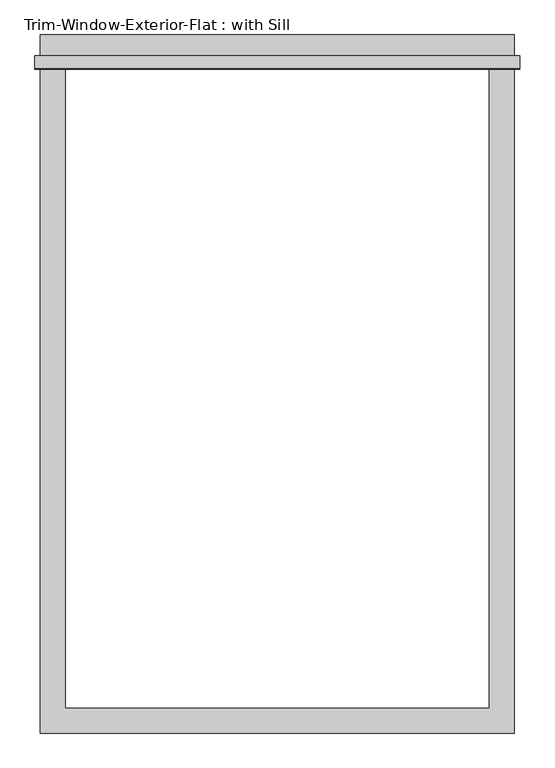
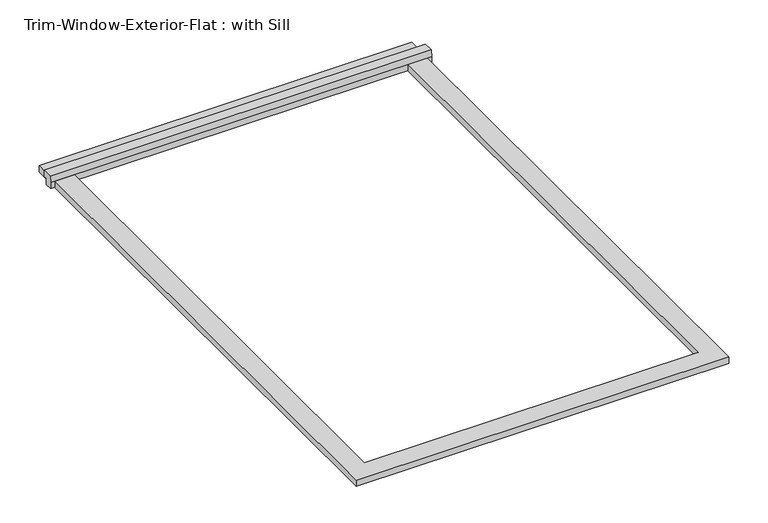
"""IFC4 building model written with IfcOpenShell, lengths in millimetres: proxy geometry, Trim-Window-Exterior-Flat : with Sill."""

from ifc_helpers import new_model, si_unit, frame, origin, origin_with_axes, place, context, project, spatial, polyline, outline, extrude, source, transform, mapped, element, save


def trim_window_exterior_flat_with_sill_c46fdb85(model_context):
    return source(origin(), model_context, "Body", "SweptSolid", [
        extrude(outline(polyline([(546.1, 1495.3823709), (-546.1, 1495.3823709), (-546.1, 1552.5323709), (546.1, 1552.5323709), (546.1, 1495.3823709)])), origin_with_axes(), (0.0, 0.0, 1.0), 19.05),
        extrude(outline(polyline([(1504.95, 38.1), (1504.95, 19.05), (1495.3823709, 19.05), (1495.3823709, 0.0), (1473.2, 0.0), (1473.2, 19.05), (1475.6580645, 38.1), (1504.95, 38.1)])), frame((-558.8, 0.0, 0.0), z_axis=(1.0, 0.0, 0.0), x_axis=(0.0, 1.0, 0.0)), (0.0, 0.0, 1.0), 1117.6),
        extrude(outline(polyline([(-546.1, -57.15), (-546.1, 1473.2), (-488.95, 1473.2), (-488.95, 0.0), (488.95, 0.0), (488.95, 1473.2), (546.1, 1473.2), (546.1, -57.15), (-546.1, -57.15)])), origin_with_axes(), (0.0, 0.0, 1.0), 19.05),
    ])


if __name__ == "__main__":
    model = new_model("IFC4")
    model_context = context("Model", 3, world=origin())
    ifc_project = project(units=[si_unit("LENGTHUNIT", "METRE", prefix="MILLI")], contexts=[model_context])
    site = spatial("IfcSite", under=ifc_project)
    building = spatial("IfcBuilding", under=site)
    placement = place(None, origin())
    trim_window_exterior_flat_with_sill_shape = trim_window_exterior_flat_with_sill_c46fdb85(model_context)
    element("IfcBuildingElementProxy", 1, Name="Trim-Window-Exterior-Flat : with Sill", ObjectType="Trim-Window-Exterior-Flat : with Sill", at=placement, inside=building, context=model_context, shape_type="MappedRepresentation", body=[
        mapped(trim_window_exterior_flat_with_sill_shape, transform((0.0, 0.0, 0.0), x_axis=(1.0, 0.0, 0.0), y_axis=(0.0, 1.0, 0.0), z_axis=(0.0, 0.0, 1.0))),
    ])
    save(model, "model.ifc")

# Revit data of these elements
# Type "Trim-Window-Exterior-Flat : with Sill"
#   Trim Width = 0' - 2 1/4"
#   Trim Thickness_Picture Frame = 0' - 1 1/4"
#   Trim Thickness_with Sill = 0' - 0 3/4"
#   Sill Thickness = 0' - 1 1/4"
#   Opening Width [instance default] = 2' - 0"
#   Opening Height [instance default] = 3' - 0"
#   Default Elevation = 4' - 0"
#   Sill = yes
#   Picture Frame = no
#   Trim Material [instance default] = none
# Element 1 (IfcBuildingElementProxy, "Trim-Window-Exterior-Flat : with Sill")
#   Opening Width = 3' - 2 1/2"
#   Opening Height = 4' - 10"
#   Trim Material = Clad - White
#   Materials on its faces: "Clad - White"
# Materials
#   "Clad - White": class "Wood", colour RGB 242 242 238, transparency 0, Cost = 0
